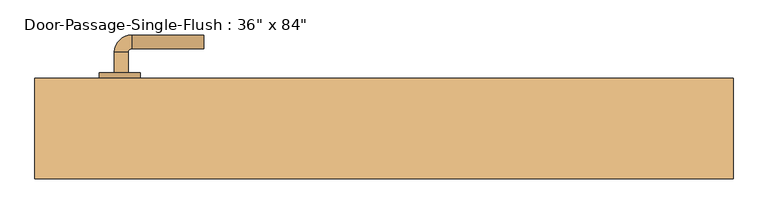
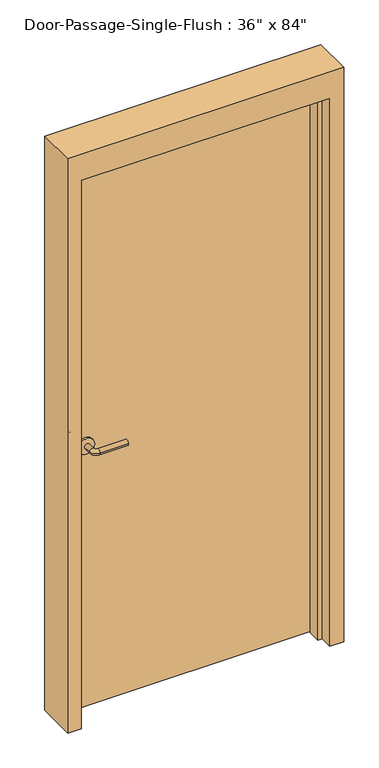
"""IFC4 building model written with IfcOpenShell, lengths in millimetres: door geometry."""

import ifcopenshell
import ifcopenshell.guid

model = None  # the IFC model being written
_history = None  # IfcOwnerHistory: only IFC2X3 demands one
_inside = {}  # id of a spatial element -> (the spatial element, [elements in it])
_under = {}  # id of a project, library or spatial element -> (it, [spatial elements below it])
_declared = {}  # id of a project -> (the project, [libraries it declares])
_typed = {}  # id of a type object -> (the type object, [elements of that type])
_made_of = {}  # id of a material, layer set ... -> (it, [elements and type objects made of it])


def new_model(schema):
    """Start an empty IFC model of exactly this schema.

    Asked for "IFC4X3", IfcOpenShell would pick the latest addendum, in which some entities
    have other attributes; the version numbers below select the first issue.
    IFC2X3 requires an IfcOwnerHistory on every rooted entity: one is made here for all.
    """
    global model, _history
    if schema == "IFC4X3":
        model = ifcopenshell.file(schema_version=(4, 3, 0, 0))
    else:
        model = ifcopenshell.file(schema=schema)
    _inside.clear()
    _under.clear()
    _declared.clear()
    _typed.clear()
    _made_of.clear()
    _history = None
    if model.schema == "IFC2X3":
        org = make("IfcOrganization", Name="unknown")
        user = make(
            "IfcPersonAndOrganization",
            ThePerson=make("IfcPerson", FamilyName="unknown"),
            TheOrganization=org,
        )
        app = make(
            "IfcApplication",
            ApplicationDeveloper=org,
            Version="unknown",
            ApplicationFullName="unknown",
            ApplicationIdentifier="unknown",
        )
        _history = make(
            "IfcOwnerHistory",
            OwningUser=user,
            OwningApplication=app,
            ChangeAction="ADDED",
            CreationDate=0,
        )
    return model


def make(cls, **values):
    """One entity of the class cls with the attributes given. An attribute that is None is left unset."""
    return model.create_entity(
        cls, **{name: value for name, value in values.items() if value is not None}
    )


def rooted(cls, **values):
    """An entity with a GlobalId (a new one), such as an element, a storey or a relation."""
    return make(cls, GlobalId=ifcopenshell.guid.new(), OwnerHistory=_history, **values)


def si_unit(unit_type, name, prefix=None):
    """IfcSIUnit, for example si_unit("LENGTHUNIT", "METRE", prefix="MILLI")."""
    return make("IfcSIUnit", UnitType=unit_type, Prefix=prefix, Name=name)


def assignment(units):
    """IfcUnitAssignment: the units of a project."""
    return None if units is None else make("IfcUnitAssignment", Units=units)


def point(xyz):
    """IfcCartesianPoint."""
    return None if xyz is None else make("IfcCartesianPoint", Coordinates=xyz)


def direction(xyz):
    """IfcDirection."""
    return None if xyz is None else make("IfcDirection", DirectionRatios=xyz)


def frame(location, z_axis=None, x_axis=None):
    """IfcAxis2Placement3D, a coordinate frame: its origin and axes. An axis left out is left unset."""
    return make(
        "IfcAxis2Placement3D",
        Location=point(location),
        Axis=direction(z_axis),
        RefDirection=direction(x_axis),
    )


def frame_2d(location, x_axis=None):
    """IfcAxis2Placement2D, a coordinate frame in the plane: its origin and x axis."""
    return make(
        "IfcAxis2Placement2D", Location=point(location), RefDirection=direction(x_axis)
    )


def origin():
    """The frame at (0, 0, 0) with its axes left unset."""
    return frame((0.0, 0.0, 0.0))


def origin_with_axes():
    """The frame at (0, 0, 0) with the z axis (0, 0, 1) and the x axis (1, 0, 0) written out."""
    return frame((0.0, 0.0, 0.0), z_axis=(0.0, 0.0, 1.0), x_axis=(1.0, 0.0, 0.0))


def place(relative_to, where):
    """IfcLocalPlacement: puts the frame where relative to a parent placement (None: the world)."""
    return make(
        "IfcLocalPlacement", PlacementRelTo=relative_to, RelativePlacement=where
    )


def context(
    kind, dimensions, precision=None, world=None, true_north=None, identifier=None
):
    """IfcGeometricRepresentationContext, for example the 3D "Model" context."""
    return make(
        "IfcGeometricRepresentationContext",
        ContextIdentifier=identifier,
        ContextType=kind,
        CoordinateSpaceDimension=dimensions,
        Precision=precision,
        WorldCoordinateSystem=world,
        TrueNorth=true_north,
    )


def project(units=None, contexts=None):
    """IfcProject with its units and contexts."""
    return rooted(
        "IfcProject",
        Name="project",
        RepresentationContexts=contexts,
        UnitsInContext=assignment(units),
    )


def spatial(cls, under=None, at=None, **own):
    """A site, building, storey or space (cls), placed at a placement, below another one or the project."""
    s = rooted(cls, ObjectPlacement=at, **own)
    if under is not None:
        _under.setdefault(under.id(), (under, []))[1].append(s)
    return s


def polyline(points):
    """IfcPolyline through the points."""
    return make("IfcPolyline", Points=[point(p) for p in points])


def circle_curve(where, radius):
    """IfcCircle in the frame where."""
    return make("IfcCircle", Position=where, Radius=radius)


def ellipse_curve(where, semi_axis1, semi_axis2):
    """IfcEllipse in the frame where."""
    return make(
        "IfcEllipse", Position=where, SemiAxis1=semi_axis1, SemiAxis2=semi_axis2
    )


def trimmed(basis, trim1, trim2, sense, master):
    """IfcTrimmedCurve: the piece of a basis curve between two trims."""
    return make(
        "IfcTrimmedCurve",
        BasisCurve=basis,
        Trim1=trim1,
        Trim2=trim2,
        SenseAgreement=sense,
        MasterRepresentation=master,
    )


def segment(curve, same_sense, transition):
    """IfcCompositeCurveSegment."""
    return make(
        "IfcCompositeCurveSegment",
        Transition=transition,
        SameSense=same_sense,
        ParentCurve=curve,
    )


def composite_curve(segments, self_intersect=None):
    """IfcCompositeCurve: segments joined end to end."""
    return make("IfcCompositeCurve", Segments=segments, SelfIntersect=self_intersect)


def outline(outer, holes=None, kind="AREA"):
    """IfcArbitraryClosedProfileDef: a profile drawn as a closed curve; with holes, ...WithVoids."""
    if holes is None:
        return make("IfcArbitraryClosedProfileDef", ProfileType=kind, OuterCurve=outer)
    return make(
        "IfcArbitraryProfileDefWithVoids",
        ProfileType=kind,
        OuterCurve=outer,
        InnerCurves=holes,
    )


def extrude(swept, where, along, depth):
    """IfcExtrudedAreaSolid: the profile swept, set in the frame where, extruded along a direction by depth."""
    return make(
        "IfcExtrudedAreaSolid",
        SweptArea=swept,
        Position=where,
        ExtrudedDirection=direction(along),
        Depth=depth,
    )


def faces_of(points, faces, orient=None, outer=None):
    """IfcFace entities. A face is a list of loops; a loop is a list of indices into points, from 0.

    orient and outer hold one flag for each loop. By default every Orientation is true, the
    first loop of a face is its IfcFaceOuterBound and the others are IfcFaceBound.
    """
    made = []
    for i, loops in enumerate(faces):
        bounds = []
        for j, loop in enumerate(loops):
            is_outer = j == 0 if outer is None else outer[i][j]
            bounds.append(
                make(
                    "IfcFaceOuterBound" if is_outer else "IfcFaceBound",
                    Bound=make("IfcPolyLoop", Polygon=[points[k] for k in loop]),
                    Orientation=True if orient is None else orient[i][j],
                )
            )
        made.append(make("IfcFace", Bounds=bounds))
    return made


def faceted_brep(points, faces, orient=None, outer=None, voids=None):
    """IfcFacetedBrep: a solid bounded by flat faces; with voids (closed shells), ...WithVoids."""
    shared = [point(p) for p in points]
    hull = make("IfcClosedShell", CfsFaces=faces_of(shared, faces, orient, outer))
    if voids is None:
        return make("IfcFacetedBrep", Outer=hull)
    return make(
        "IfcFacetedBrepWithVoids",
        Outer=hull,
        Voids=[
            make(cls, CfsFaces=faces_of(shared, fs, o, b)) for cls, fs, o, b in voids
        ],
    )


def shape(context_of_items, identifier, shape_type, items):
    """IfcShapeRepresentation: the items that make up one representation, for example the "Body"."""
    return make(
        "IfcShapeRepresentation",
        ContextOfItems=context_of_items,
        RepresentationIdentifier=identifier,
        RepresentationType=shape_type,
        Items=items,
    )


def source(mapping_origin, context_of_items, identifier, shape_type, items):
    """IfcRepresentationMap: a shape defined once, which mapped items show again and again."""
    return make(
        "IfcRepresentationMap",
        MappingOrigin=mapping_origin,
        MappedRepresentation=shape(context_of_items, identifier, shape_type, items),
    )


def transform(
    local_origin,
    x_axis=None,
    y_axis=None,
    z_axis=None,
    scale=None,
    scale2=None,
    scale3=None,
    uniform=True,
):
    """IfcCartesianTransformationOperator3D, or its non-uniform kind. x_axis, y_axis, z_axis: its Axis1, 2, 3."""
    if uniform:
        return make(
            "IfcCartesianTransformationOperator3D",
            Axis1=direction(x_axis),
            Axis2=direction(y_axis),
            LocalOrigin=point(local_origin),
            Scale=scale,
            Axis3=direction(z_axis),
        )
    return make(
        "IfcCartesianTransformationOperator3DnonUniform",
        Axis1=direction(x_axis),
        Axis2=direction(y_axis),
        LocalOrigin=point(local_origin),
        Scale=scale,
        Axis3=direction(z_axis),
        Scale2=scale2,
        Scale3=scale3,
    )


def mapped(mapping_source, mapping_target):
    """IfcMappedItem: shows the shape of a source again, moved by a transform."""
    return make(
        "IfcMappedItem", MappingSource=mapping_source, MappingTarget=mapping_target
    )


def made_of(thing, what):
    """Note that an element or type object is made of a material, layer set ...; save() writes the relation."""
    if what is not None:
        _made_of.setdefault(what.id(), (what, []))[1].append(thing)
    return thing


def element(
    cls,
    number,
    at=None,
    inside=None,
    cuts=None,
    type_object=None,
    material=None,
    context=None,
    identifier="Body",
    shape_type=None,
    held_by="IfcProductDefinitionShape",
    body=None,
    shapes=None,
    **own,
):
    """One element of the class cls, such as IfcWall. Its Tag is "e" and its number.

    at: its placement. inside: the storey or other place that contains it. cuts: it is an
    opening in that element (IfcRelVoidsElement). A single representation is given by context,
    identifier, shape_type and body (its items); several are given by shapes. held_by: the class
    of the entity that holds the representations. save() writes the other relations.
    """
    e = rooted(cls, Tag="e%d" % number, ObjectPlacement=at, **own)
    if body is not None:
        shapes = [shape(context, identifier, shape_type, body)]
    if shapes is not None:
        e.Representation = make(held_by, Representations=shapes)
    if inside is not None:
        _inside.setdefault(inside.id(), (inside, []))[1].append(e)
    if cuts is not None:
        rooted(
            "IfcRelVoidsElement", RelatingBuildingElement=cuts, RelatedOpeningElement=e
        )
    if type_object is not None:
        _typed.setdefault(type_object.id(), (type_object, []))[1].append(e)
    return made_of(e, material)


def aggregate(whole, parts):
    """IfcRelAggregates: a whole, such as a stair, and the parts it consists of."""
    return rooted("IfcRelAggregates", RelatingObject=whole, RelatedObjects=parts)


def save(model, path):
    """Write the relations noted so far, then the file.

    IfcRelAggregates (storeys below a building ...), IfcRelContainedInSpatialStructure (elements
    in a storey), IfcRelDefinesByType, IfcRelAssociatesMaterial and IfcRelDeclares: one each for
    every whole, place, type object, material and project.
    """
    for whole, parts in _under.values():
        aggregate(whole, parts)
    for where, things in _inside.values():
        rooted(
            "IfcRelContainedInSpatialStructure",
            RelatedElements=things,
            RelatingStructure=where,
        )
    for kind, things in _typed.values():
        rooted("IfcRelDefinesByType", RelatedObjects=things, RelatingType=kind)
    for what, things in _made_of.values():
        rooted("IfcRelAssociatesMaterial", RelatedObjects=things, RelatingMaterial=what)
    for by, libraries in _declared.values():
        rooted("IfcRelDeclares", RelatingContext=by, RelatedDefinitions=libraries)
    model.write(path)


def plane_surface(at):
    """IfcPlane: the flat surface through the origin of the frame at, square to its z axis."""
    return make("IfcPlane", Position=at)


def cylinder_surface(at, radius):
    """IfcCylindricalSurface: all points at the distance radius from the z axis of the frame at."""
    return make("IfcCylindricalSurface", Position=at, Radius=radius)


def revolved_surface(curve, axis_point, axis_direction):
    """IfcSurfaceOfRevolution: the curve turned about the line through axis_point along axis_direction."""
    return make(
        "IfcSurfaceOfRevolution",
        SweptCurve=make("IfcArbitraryOpenProfileDef", ProfileType="CURVE", Curve=curve),
        AxisPosition=make("IfcAxis1Placement", Location=point(axis_point), Axis=direction(axis_direction)),
    )


def advanced_brep(points, edges, surfaces, faces):
    """IfcAdvancedBrep: a solid bounded by faces that lie on surfaces and meet in shared edges.

    An edge is (start, end): straight between two places in points (the first is 0);
    or (start, end, curve); or (start, end, curve, False) where it runs against its curve.
    A face is (place in surfaces, loops), or (place, loops, False) where it looks against
    its surface's normal. A loop lists edges by number (the first is 1), with a minus sign
    where the edge is run from its end to its start. The first loop is the outer one.
    """
    corners = [point(p) for p in points]
    vertices = [make("IfcVertexPoint", VertexGeometry=c) for c in corners]
    made = []
    for start, end, *more in edges:
        made.append(
            make(
                "IfcEdgeCurve",
                EdgeStart=vertices[start],
                EdgeEnd=vertices[end],
                EdgeGeometry=more[0] if more else make("IfcPolyline", Points=[corners[start], corners[end]]),
                SameSense=more[1] if len(more) > 1 else True,
            )
        )
    hull = []
    for where, loops, *sense in faces:
        bounds = []
        for j, loop in enumerate(loops):
            ring = [make("IfcOrientedEdge", EdgeElement=made[abs(k) - 1], Orientation=k > 0) for k in loop]
            bounds.append(
                make(
                    "IfcFaceOuterBound" if j == 0 else "IfcFaceBound",
                    Bound=make("IfcEdgeLoop", EdgeList=ring),
                    Orientation=True,
                )
            )
        hull.append(make("IfcAdvancedFace", Bounds=bounds, FaceSurface=surfaces[where], SameSense=sense[0] if sense else True))
    return make("IfcAdvancedBrep", Outer=make("IfcClosedShell", CfsFaces=hull))


def door_87fe937e(model_context):
    return source(origin(), model_context, "Body", "SolidModel", [
        advanced_brep(
        [(-392.190625, 25.3375, 1016.0), (-372.190625, 25.3375, 1016.0), (-372.190625, -4.6625, 1016.0), (-392.190625, -4.6625, 1016.0), (-367.190625, -9.6625, 1016.0), (-367.190625, -29.6625, 1016.0), (-262.190625, -29.6625, 1016.0), (-262.190625, -9.6625, 1016.0)],
        [
            (0, 1, circle_curve(frame((-382.190625, 25.3375, 1016.0), z_axis=(0.0, 1.0, 0.0), x_axis=(1.0, 0.0, 0.0)), 10.0)),
            (1, 0, circle_curve(frame((-382.190625, 25.3375, 1016.0), z_axis=(0.0, 1.0, 0.0), x_axis=(1.0, 0.0, 0.0)), 10.0)),
            (1, 2),
            (2, 3, circle_curve(frame((-382.190625, -4.6625, 1016.0), z_axis=(0.0, 1.0, 0.0), x_axis=(1.0, 0.0, 0.0)), 10.0)),
            (3, 0),
            (3, 2, circle_curve(frame((-382.190625, -4.6625, 1016.0), z_axis=(0.0, 1.0, 0.0), x_axis=(1.0, 0.0, 0.0)), 10.0)),
            (4, 5, circle_curve(frame((-367.190625, -19.6625, 1016.0), z_axis=(-1.0, 0.0, 0.0), x_axis=(0.0, 1.0, 0.0)), 10.0)),
            (5, 3, circle_curve(frame((-367.190625, -4.6625, 1016.0), z_axis=(0.0, 0.0, -1.0), x_axis=(-1.0, 0.0, 0.0)), 25.0)),
            (2, 4, circle_curve(frame((-367.190625, -4.6625, 1016.0), z_axis=(0.0, 0.0, 1.0), x_axis=(-1.0, 0.0, 0.0)), 5.0)),
            (5, 4, circle_curve(frame((-367.190625, -19.6625, 1016.0), z_axis=(-1.0, 0.0, 0.0), x_axis=(0.0, 1.0, 0.0)), 10.0)),
            (6, 7, circle_curve(frame((-262.190625, -19.6625, 1016.0), z_axis=(1.0, 0.0, 0.0), x_axis=(0.0, 1.0, 0.0)), 10.0)),
            (7, 6, circle_curve(frame((-262.190625, -19.6625, 1016.0), z_axis=(1.0, 0.0, 0.0), x_axis=(0.0, 1.0, 0.0)), 10.0)),
            (4, 7),
            (6, 5),
        ],
        [
            plane_surface(frame((-382.190625, 25.3375, 1016.0), z_axis=(0.0, 1.0, 0.0), x_axis=(0.0, 0.0, 1.0))),
            cylinder_surface(frame((-382.190625, 25.3375, 1016.0), z_axis=(0.0, 1.0, 0.0), x_axis=(1.0, 0.0, 0.0)), 10.0),
            revolved_surface(trimmed(ellipse_curve(frame((-382.190625, -4.6625, 1016.0), z_axis=(0.0, -1.0, 0.0), x_axis=(1.0, 0.0, 0.0)), 10.0, 10.0), [point((-392.190625, -4.6625, 1016.0))], [point((-372.190625, -4.6625, 1016.0))], True, "CARTESIAN"), (-367.190625, -4.6625, 1016.0), (0.0, 0.0, -1.0)),
            revolved_surface(trimmed(ellipse_curve(frame((-382.190625, -4.6625, 1016.0), z_axis=(0.0, -1.0, 0.0), x_axis=(1.0, 0.0, 0.0)), 10.0, 10.0), [point((-372.190625, -4.6625, 1016.0))], [point((-392.190625, -4.6625, 1016.0))], True, "CARTESIAN"), (-367.190625, -4.6625, 1016.0), (0.0, 0.0, -1.0)),
            plane_surface(frame((-262.190625, -19.6625, 1016.0), z_axis=(1.0, 0.0, 0.0), x_axis=(0.0, 0.0, 1.0))),
            cylinder_surface(frame((-367.190625, -19.6625, 1016.0), z_axis=(-1.0, 0.0, 0.0), x_axis=(0.0, 1.0, 0.0)), 10.0),
        ],
        [
            (0, [[1, 2]]),
            (1, [[3, 4, 5, -2]]),
            (1, [[-5, 6, -3, -1]]),
            (2, [[7, 8, -4, 9]]),
            (3, [[10, -9, -6, -8]]),
            (4, [[11, 12]]),
            (5, [[13, -11, 14, -7]]),
            (5, [[-14, -12, -13, -10]]),
        ],
    ),
        extrude(outline(composite_curve([segment(trimmed(circle_curve(frame_2d((1016.0, -384.690625)), 30.0), [point((1016.0, -414.690625))], [point((1016.0, -354.690625))], False, "CARTESIAN"), True, "CONTINUOUS"), segment(trimmed(circle_curve(frame_2d((1016.0, -384.690625)), 30.0), [point((1016.0, -354.690625))], [point((1016.0, -414.690625))], False, "CARTESIAN"), True, "CONTINUOUS")], self_intersect=False)), frame((0.0, 25.3375, 0.0), z_axis=(0.0, 1.0, 0.0), x_axis=(0.0, 0.0, 1.0)), (0.0, 0.0, 1.0), 8.0),
        advanced_brep(
        [(-392.190625, 85.7875, 1016.0), (-372.190625, 85.7875, 1016.0), (-392.190625, 115.7875, 1016.0), (-372.190625, 115.7875, 1016.0), (-367.190625, 120.7875, 1016.0), (-367.190625, 140.7875, 1016.0), (-262.190625, 140.7875, 1016.0), (-262.190625, 120.7875, 1016.0)],
        [
            (0, 1, circle_curve(frame((-382.190625, 85.7875, 1016.0), z_axis=(0.0, -1.0, 0.0), x_axis=(1.0, 0.0, 0.0)), 10.0)),
            (1, 0, circle_curve(frame((-382.190625, 85.7875, 1016.0), z_axis=(0.0, -1.0, 0.0), x_axis=(1.0, 0.0, 0.0)), 10.0)),
            (0, 2),
            (2, 3, circle_curve(frame((-382.190625, 115.7875, 1016.0), z_axis=(0.0, -1.0, 0.0), x_axis=(1.0, 0.0, 0.0)), 10.0)),
            (3, 1),
            (3, 2, circle_curve(frame((-382.190625, 115.7875, 1016.0), z_axis=(0.0, -1.0, 0.0), x_axis=(1.0, 0.0, 0.0)), 10.0)),
            (4, 3, circle_curve(frame((-367.190625, 115.7875, 1016.0), z_axis=(0.0, 0.0, 1.0), x_axis=(-1.0, 0.0, 0.0)), 5.0)),
            (2, 5, circle_curve(frame((-367.190625, 115.7875, 1016.0), z_axis=(0.0, 0.0, -1.0), x_axis=(-1.0, 0.0, 0.0)), 25.0)),
            (5, 4, circle_curve(frame((-367.190625, 130.7875, 1016.0), z_axis=(-1.0, 0.0, 0.0), x_axis=(0.0, -1.0, 0.0)), 10.0)),
            (4, 5, circle_curve(frame((-367.190625, 130.7875, 1016.0), z_axis=(-1.0, 0.0, 0.0), x_axis=(0.0, -1.0, 0.0)), 10.0)),
            (6, 7, circle_curve(frame((-262.190625, 130.7875, 1016.0), z_axis=(1.0, 0.0, 0.0), x_axis=(0.0, -1.0, 0.0)), 10.0)),
            (7, 6, circle_curve(frame((-262.190625, 130.7875, 1016.0), z_axis=(1.0, 0.0, 0.0), x_axis=(0.0, -1.0, 0.0)), 10.0)),
            (5, 6),
            (7, 4),
        ],
        [
            plane_surface(frame((-382.190625, 85.7875, 1016.0), z_axis=(0.0, -1.0, 0.0), x_axis=(0.0, 0.0, 1.0))),
            cylinder_surface(frame((-382.190625, 85.7875, 1016.0), z_axis=(0.0, -1.0, 0.0), x_axis=(1.0, 0.0, 0.0)), 10.0),
            revolved_surface(trimmed(ellipse_curve(frame((-382.190625, 115.7875, 1016.0), z_axis=(0.0, -1.0, 0.0), x_axis=(1.0, 0.0, 0.0)), 10.0, 10.0), [point((-392.190625, 115.7875, 1016.0))], [point((-372.190625, 115.7875, 1016.0))], True, "CARTESIAN"), (-367.190625, 115.7875, 1016.0), (0.0, 0.0, -1.0)),
            revolved_surface(trimmed(ellipse_curve(frame((-382.190625, 115.7875, 1016.0), z_axis=(0.0, -1.0, 0.0), x_axis=(1.0, 0.0, 0.0)), 10.0, 10.0), [point((-372.190625, 115.7875, 1016.0))], [point((-392.190625, 115.7875, 1016.0))], True, "CARTESIAN"), (-367.190625, 115.7875, 1016.0), (0.0, 0.0, -1.0)),
            plane_surface(frame((-262.190625, 130.7875, 1016.0), z_axis=(1.0, 0.0, 0.0), x_axis=(0.0, 0.0, 1.0))),
            cylinder_surface(frame((-367.190625, 130.7875, 1016.0), z_axis=(-1.0, 0.0, 0.0), x_axis=(0.0, -1.0, 0.0)), 10.0),
        ],
        [
            (0, [[1, 2]]),
            (1, [[-1, 3, 4, 5]]),
            (1, [[-2, -5, 6, -3]]),
            (2, [[7, -4, 8, 9]]),
            (3, [[-8, -6, -7, 10]]),
            (4, [[11, 12]]),
            (5, [[-9, 13, -12, 14]]),
            (5, [[-10, -14, -11, -13]]),
        ],
    ),
        extrude(outline(composite_curve([segment(trimmed(circle_curve(frame_2d((1016.0, -384.690625)), 30.0), [point((1016.0, -414.690625))], [point((1016.0, -354.690625))], False, "CARTESIAN"), True, "CONTINUOUS"), segment(trimmed(circle_curve(frame_2d((1016.0, -384.690625)), 30.0), [point((1016.0, -354.690625))], [point((1016.0, -414.690625))], False, "CARTESIAN"), True, "CONTINUOUS")], self_intersect=False)), frame((0.0, 77.7875, 0.0), z_axis=(0.0, 1.0, 0.0), x_axis=(0.0, 0.0, 1.0)), (0.0, 0.0, 1.0), 8.0),
        faceted_brep([(457.2, 28.575, 0.0), (457.2, 77.7875, 0.0), (508.0, 77.7875, 0.0), (508.0, -68.2625, 0.0), (457.2, -68.2625, 0.0), (457.2, -19.05, 0.0), (441.325, -19.05, 0.0), (441.325, 28.575, 0.0), (457.2, 28.575, 2133.6), (457.2, 77.7875, 2133.6), (-457.2, 77.7875, 2133.6), (-457.2, 77.7875, 0.0), (-508.0, 77.7875, 0.0), (-508.0, 77.7875, 2235.2), (508.0, 77.7875, 2235.2), (508.0, -68.2625, 2235.2), (-508.0, -68.2625, 2235.2), (-508.0, -68.2625, 0.0), (-457.2, -68.2625, 0.0), (-457.2, -68.2625, 2133.6), (457.2, -68.2625, 2133.6), (457.2, -19.05, 2133.6), (-457.2, -19.05, 2133.6), (-457.2, -19.05, 0.0), (-441.325, -19.05, 0.0), (-441.325, -19.05, 2117.725), (441.325, -19.05, 2117.725), (441.325, 28.575, 2117.725), (-441.325, 28.575, 2117.725), (-441.325, 28.575, 0.0), (-457.2, 28.575, 0.0), (-457.2, 28.575, 2133.6)], [[[0, 1, 2, 3, 4, 5, 6, 7]], [[1, 0, 8, 9]], [[2, 1, 9, 10, 11, 12, 13, 14]], [[3, 2, 14, 15]], [[4, 3, 15, 16, 17, 18, 19, 20]], [[5, 4, 20, 21]], [[6, 5, 21, 22, 23, 24, 25, 26]], [[7, 6, 26, 27]], [[0, 7, 27, 28, 29, 30, 31, 8]], [[9, 8, 31, 10]], [[20, 19, 22, 21]], [[26, 25, 28, 27]], [[12, 11, 30, 29, 24, 23, 18, 17]], [[11, 10, 31, 30]], [[13, 12, 17, 16]], [[19, 18, 23, 22]], [[25, 24, 29, 28]], [[15, 14, 13, 16]]]),
        extrude(outline(polyline([(457.2, 33.3375), (-457.2, 33.3375), (-457.2, 77.7875), (457.2, 77.7875), (457.2, 33.3375)])), origin_with_axes(), (0.0, 0.0, 1.0), 2133.6),
    ])


if __name__ == "__main__":
    model = new_model("IFC4")
    model_context = context("Model", 3, world=origin())
    ifc_project = project(units=[si_unit("LENGTHUNIT", "METRE", prefix="MILLI")], contexts=[model_context])
    site = spatial("IfcSite", under=ifc_project)
    building = spatial("IfcBuilding", under=site)
    placement = place(None, origin())
    door_shape = door_87fe937e(model_context)
    element("IfcDoor", 1, ObjectType="Door-Passage-Single-Flush : 36\" x 84\"", at=placement, inside=building, context=model_context, shape_type="MappedRepresentation", body=[
        mapped(door_shape, transform((0.0, 0.0, 0.0), x_axis=(1.0, 0.0, 0.0), y_axis=(0.0, 1.0, 0.0), z_axis=(0.0, 0.0, 1.0))),
    ])
    save(model, "model.ifc")

# Revit data of these elements
# Type "Door-Passage-Single-Flush : 36\" x 84\""
#   Type Mark = "1"
#   Assembly Code = "B2030200"
#   Analytic Construction = "Wooden"
#   Thickness = 0' - 1 3/4"
#   Thermal Resistance (R) = 2.5876 (h·ft²·°F)/BTU
#   Swing Angle [instance default] = 90.00°
#   Strike Height = 3' - 4"
#   Rough Width [instance default] = 3' - 4"
#   Rough Height [instance default] = 7' - 4"
#   MF Opening Height [instance default] = 0' - 4"
#   MF Opening Width [instance default] = 0' - 4"
#   Inset Calculate [instance default] = 0' - 4"
#   Masonry Inset [instance default] = 0' - 1"
#   Height = 7' - 0"
#   Width = 3' - 0"
#   Heat Transfer Coefficient (U) = 0.3865 BTU/(h·ft²·°F)
#   Masonry Frame Depth = 0' - 5 3/4"
#   Define Thermal Properties by = 1
#   Masonry Frame [instance default] = yes
#   Function = 1
#   Dry Wall Frame [instance default] = no
#   Panel Material = Wood - Birch
#   Frame Material = Metal - Paint Finish - Grey
#   Door Handle Material = Aluminum
#   Visual Light Transmittance = 0
#   Solar Heat Gain Coefficient = 0
#   Wall Closure = (empty or 0)
# Element 1 (IfcDoor, "Door-Passage-Single-Flush : 36\" x 84\"")
#   Materials on its faces: "Aluminum", "Metal - Paint Finish - Grey", "Wood - Birch"
# Materials
#   "Wood - Birch": class "Wood", colour RGB 166 116 52, transparency 0, Cost = 0
#   "Metal - Paint Finish - Grey": class "Paint", colour RGB 104 104 104, transparency 0, Cost = 0
#   "Aluminum": class "Metal", colour RGB 247 247 247, transparency 0, Description = "Aluminum 6061", Cost = 0
